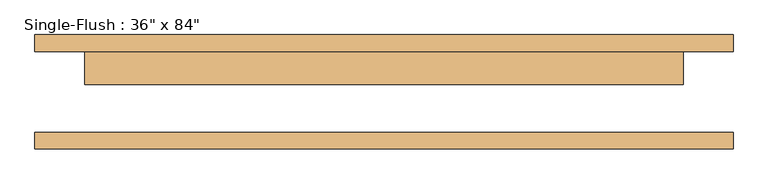
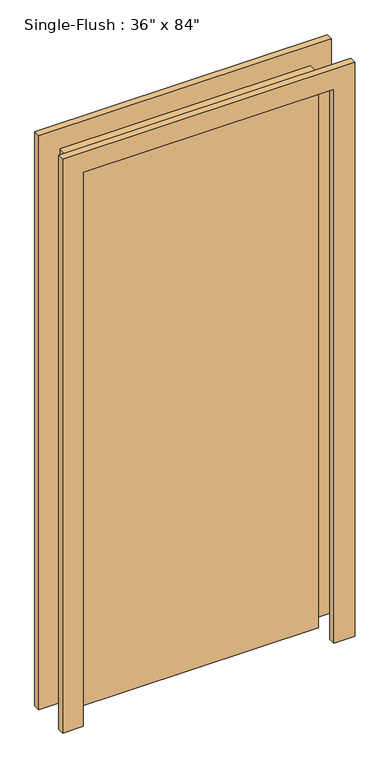
"""IFC4 building model written with IfcOpenShell, lengths in millimetres: door geometry."""

from ifc_helpers import new_model, si_unit, frame, origin, origin_with_axes, place, context, project, spatial, polyline, outline, extrude, source, transform, mapped, element, save


def door_88503111(model_context):
    return source(origin(), model_context, "Body", "SweptSolid", [
        extrude(outline(polyline([(2209.8, -533.4), (0.0, -533.4), (0.0, -457.2), (2133.6, -457.2), (2133.6, 457.2), (0.0, 457.2), (0.0, 533.4), (2209.8, 533.4), (2209.8, -533.4)])), frame((0.0, 61.9125, 0.0), z_axis=(0.0, 1.0, 0.0), x_axis=(0.0, 0.0, 1.0)), (0.0, 0.0, 1.0), 25.4),
        extrude(outline(polyline([(2209.8, 533.4), (2209.8, -533.4), (0.0, -533.4), (0.0, -457.2), (2133.6, -457.2), (2133.6, 457.2), (0.0, 457.2), (0.0, 533.4), (2209.8, 533.4)])), frame((0.0, -87.3125, 0.0), z_axis=(0.0, 1.0, 0.0), x_axis=(0.0, 0.0, 1.0)), (0.0, 0.0, 1.0), 25.4),
        extrude(outline(polyline([(457.2, 11.1125), (-457.2, 11.1125), (-457.2, 61.9125), (457.2, 61.9125), (457.2, 11.1125)])), origin_with_axes(), (0.0, 0.0, 1.0), 2133.6),
    ])


if __name__ == "__main__":
    model = new_model("IFC4")
    model_context = context("Model", 3, world=origin())
    ifc_project = project(units=[si_unit("LENGTHUNIT", "METRE", prefix="MILLI")], contexts=[model_context])
    site = spatial("IfcSite", under=ifc_project)
    building = spatial("IfcBuilding", under=site)
    placement = place(None, origin())
    door_shape = door_88503111(model_context)
    element("IfcDoor", 1, ObjectType="Single-Flush : 36\" x 84\"", at=placement, inside=building, context=model_context, shape_type="MappedRepresentation", body=[
        mapped(door_shape, transform((0.0, 0.0, 0.0), x_axis=(1.0, 0.0, 0.0), y_axis=(0.0, 1.0, 0.0), z_axis=(0.0, 0.0, 1.0))),
    ])
    save(model, "model.ifc")

# Revit data of these elements
# Type "Single-Flush : 36\" x 84\""
#   Type Mark = "1"
#   Assembly Code = "C1020"
#   Thickness = 0' - 2"
#   Height = 7' - 0"
#   Trim Projection Ext = 0' - 1"
#   Trim Projection Int = 0' - 1"
#   Trim Width = 0' - 3"
#   Width = 3' - 0"
#   Door Material = none
#   Frame Material = none
#   Function = (empty or 0)
#   Wall Closure = (empty or 0)
